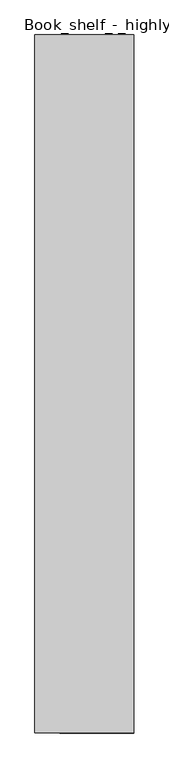
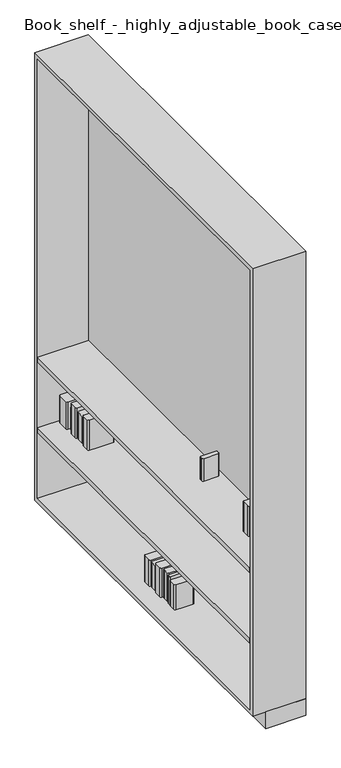
"""IFC4 building model written with IfcOpenShell, lengths in millimetres: furniture geometry."""

from ifc_helpers import new_model, si_unit, point, frame, frame_2d, origin, origin_with_axes, place, context, project, spatial, polyline, circle_curve, trimmed, segment, composite_curve, outline, extrude, source, transform, mapped, element, save


def furniture_61dade96(model_context):
    return source(origin(), model_context, "Body", "SweptSolid", [
        extrude(outline(composite_curve([segment(polyline([(-174.9979766, 273.5343096), (-174.9979766, 313.4842776)]), True, "CONTINUOUS"), segment(trimmed(circle_curve(frame_2d((-168.6479766, 313.4842776)), 6.35), [point((-174.9979766, 313.4842776))], [point((-168.6479766, 319.8342776))], False, "CARTESIAN"), True, "CONTINUOUS"), segment(polyline([(-168.6479766, 319.8342776), (-44.45, 319.8342776)]), True, "CONTINUOUS"), segment(trimmed(circle_curve(frame_2d((-44.45, 313.4842776)), 6.35), [point((-44.45, 319.8342776))], [point((-38.1, 313.4842776))], False, "CARTESIAN"), True, "CONTINUOUS"), segment(polyline([(-38.1, 313.4842776), (-38.1, 273.5343096)]), True, "CONTINUOUS"), segment(trimmed(circle_curve(frame_2d((-44.45, 273.5343096)), 6.35), [point((-38.1, 273.5343096))], [point((-44.45, 267.1843096))], False, "CARTESIAN"), True, "CONTINUOUS"), segment(polyline([(-44.45, 267.1843096), (-168.6479766, 267.1843096)]), True, "CONTINUOUS"), segment(trimmed(circle_curve(frame_2d((-168.6479766, 273.5343096)), 6.35), [point((-168.6479766, 267.1843096))], [point((-174.9979766, 273.5343096))], False, "CARTESIAN"), True, "CONTINUOUS")], self_intersect=False)), frame((0.0, 0.0, 977.8), z_axis=(0.0, 0.0, 1.0), x_axis=(1.0, 0.0, 0.0)), (0.0, 0.0, 1.0), 181.3914823),
        extrude(outline(composite_curve([segment(polyline([(-134.504595, 796.0843096), (-134.504595, 808.7843096)]), True, "CONTINUOUS"), segment(trimmed(circle_curve(frame_2d((-128.154595, 808.7843096)), 6.35), [point((-134.504595, 808.7843096))], [point((-128.154595, 815.1343096))], False, "CARTESIAN"), True, "CONTINUOUS"), segment(polyline([(-128.154595, 815.1343096), (-44.45, 815.1343096)]), True, "CONTINUOUS"), segment(trimmed(circle_curve(frame_2d((-44.45, 808.7843096)), 6.35), [point((-44.45, 815.1343096))], [point((-38.1, 808.7843096))], False, "CARTESIAN"), True, "CONTINUOUS"), segment(polyline([(-38.1, 808.7843096), (-38.1, 796.0843096)]), True, "CONTINUOUS"), segment(trimmed(circle_curve(frame_2d((-44.45, 796.0843096)), 6.35), [point((-38.1, 796.0843096))], [point((-44.45, 789.7343096))], False, "CARTESIAN"), True, "CONTINUOUS"), segment(polyline([(-44.45, 789.7343096), (-128.154595, 789.7343096)]), True, "CONTINUOUS"), segment(trimmed(circle_curve(frame_2d((-128.154595, 796.0843096)), 6.35), [point((-128.154595, 789.7343096))], [point((-134.504595, 796.0843096))], False, "CARTESIAN"), True, "CONTINUOUS")], self_intersect=False)), frame((0.0, 0.0, 977.8), z_axis=(0.0, 0.0, 1.0), x_axis=(1.0, 0.0, 0.0)), (0.0, 0.0, 1.0), 135.8183694),
        extrude(outline(composite_curve([segment(polyline([(-174.9979766, 154.4873472), (-174.9979766, 194.4373151)]), True, "CONTINUOUS"), segment(trimmed(circle_curve(frame_2d((-168.6479766, 194.4373151)), 6.35), [point((-174.9979766, 194.4373151))], [point((-168.6479766, 200.7873151))], False, "CARTESIAN"), True, "CONTINUOUS"), segment(polyline([(-168.6479766, 200.7873151), (-44.45, 200.7873151)]), True, "CONTINUOUS"), segment(trimmed(circle_curve(frame_2d((-44.45, 194.4373151)), 6.35), [point((-44.45, 200.7873151))], [point((-38.1, 194.4373151))], False, "CARTESIAN"), True, "CONTINUOUS"), segment(polyline([(-38.1, 194.4373151), (-38.1, 154.4873472)]), True, "CONTINUOUS"), segment(trimmed(circle_curve(frame_2d((-44.45, 154.4873472)), 6.35), [point((-38.1, 154.4873472))], [point((-44.45, 148.1373472))], False, "CARTESIAN"), True, "CONTINUOUS"), segment(polyline([(-44.45, 148.1373472), (-168.6479766, 148.1373472)]), True, "CONTINUOUS"), segment(trimmed(circle_curve(frame_2d((-168.6479766, 154.4873472)), 6.35), [point((-168.6479766, 148.1373472))], [point((-174.9979766, 154.4873472))], False, "CARTESIAN"), True, "CONTINUOUS")], self_intersect=False)), frame((0.0, 0.0, 977.8), z_axis=(0.0, 0.0, 1.0), x_axis=(1.0, 0.0, 0.0)), (0.0, 0.0, 1.0), 181.3914823),
        extrude(outline(composite_curve([segment(polyline([(-148.9022418, 213.6855624), (-148.9022418, 254.1898725)]), True, "CONTINUOUS"), segment(trimmed(circle_curve(frame_2d((-142.5522418, 254.1898725)), 6.35), [point((-148.9022418, 254.1898725))], [point((-142.5522418, 260.5398725))], False, "CARTESIAN"), True, "CONTINUOUS"), segment(polyline([(-142.5522418, 260.5398725), (-44.45, 260.5398725)]), True, "CONTINUOUS"), segment(trimmed(circle_curve(frame_2d((-44.45, 254.1898725)), 6.35), [point((-44.45, 260.5398725))], [point((-38.1, 254.1898725))], False, "CARTESIAN"), True, "CONTINUOUS"), segment(polyline([(-38.1, 254.1898725), (-38.1, 213.6855624)]), True, "CONTINUOUS"), segment(trimmed(circle_curve(frame_2d((-44.45, 213.6855624)), 6.35), [point((-38.1, 213.6855624))], [point((-44.45, 207.3355624))], False, "CARTESIAN"), True, "CONTINUOUS"), segment(polyline([(-44.45, 207.3355624), (-142.5522418, 207.3355624)]), True, "CONTINUOUS"), segment(trimmed(circle_curve(frame_2d((-142.5522418, 213.6855624)), 6.35), [point((-142.5522418, 207.3355624))], [point((-148.9022418, 213.6855624))], False, "CARTESIAN"), True, "CONTINUOUS")], self_intersect=False)), frame((0.0, 0.0, 977.8), z_axis=(0.0, 0.0, 1.0), x_axis=(1.0, 0.0, 0.0)), (0.0, 0.0, 1.0), 163.8466778),
        extrude(outline(composite_curve([segment(polyline([(-155.6511388, 44.45), (-155.6511388, 48.7119243)]), True, "CONTINUOUS"), segment(trimmed(circle_curve(frame_2d((-149.3011388, 48.7119243)), 6.35), [point((-155.6511388, 48.7119243))], [point((-149.3011388, 55.0619243))], False, "CARTESIAN"), True, "CONTINUOUS"), segment(polyline([(-149.3011388, 55.0619243), (-44.45, 55.0619243)]), True, "CONTINUOUS"), segment(trimmed(circle_curve(frame_2d((-44.45, 48.7119243)), 6.35), [point((-44.45, 55.0619243))], [point((-38.1, 48.7119243))], False, "CARTESIAN"), True, "CONTINUOUS"), segment(polyline([(-38.1, 48.7119243), (-38.1, 44.45)]), True, "CONTINUOUS"), segment(trimmed(circle_curve(frame_2d((-44.45, 44.45)), 6.35), [point((-38.1, 44.45))], [point((-44.45, 38.1))], False, "CARTESIAN"), True, "CONTINUOUS"), segment(polyline([(-44.45, 38.1), (-149.3011388, 38.1)]), True, "CONTINUOUS"), segment(trimmed(circle_curve(frame_2d((-149.3011388, 44.45)), 6.35), [point((-149.3011388, 38.1))], [point((-155.6511388, 44.45))], False, "CARTESIAN"), True, "CONTINUOUS")], self_intersect=False)), frame((0.0, 0.0, 977.8), z_axis=(0.0, 0.0, 1.0), x_axis=(1.0, 0.0, 0.0)), (0.0, 0.0, 1.0), 166.2690481),
        extrude(outline(composite_curve([segment(polyline([(-191.8289872, 93.2744988), (-191.8289872, 133.2244668)]), True, "CONTINUOUS"), segment(trimmed(circle_curve(frame_2d((-185.4789872, 133.2244668)), 6.35), [point((-191.8289872, 133.2244668))], [point((-185.4789872, 139.5744668))], False, "CARTESIAN"), True, "CONTINUOUS"), segment(polyline([(-185.4789872, 139.5744668), (-44.45, 139.5744668)]), True, "CONTINUOUS"), segment(trimmed(circle_curve(frame_2d((-44.45, 133.2244668)), 6.35), [point((-44.45, 139.5744668))], [point((-38.1, 133.2244668))], False, "CARTESIAN"), True, "CONTINUOUS"), segment(polyline([(-38.1, 133.2244668), (-38.1, 93.2744988)]), True, "CONTINUOUS"), segment(trimmed(circle_curve(frame_2d((-44.45, 93.2744988)), 6.35), [point((-38.1, 93.2744988))], [point((-44.45, 86.9244988))], False, "CARTESIAN"), True, "CONTINUOUS"), segment(polyline([(-44.45, 86.9244988), (-185.4789872, 86.9244988)]), True, "CONTINUOUS"), segment(trimmed(circle_curve(frame_2d((-185.4789872, 93.2744988)), 6.35), [point((-185.4789872, 86.9244988))], [point((-191.8289872, 93.2744988))], False, "CARTESIAN"), True, "CONTINUOUS")], self_intersect=False)), frame((0.0, 0.0, 977.8), z_axis=(0.0, 0.0, 1.0), x_axis=(1.0, 0.0, 0.0)), (0.0, 0.0, 1.0), 148.7566688),
        extrude(outline(composite_curve([segment(polyline([(-177.3825869, 67.874514), (-177.3825869, 75.2798723)]), True, "CONTINUOUS"), segment(trimmed(circle_curve(frame_2d((-171.0325869, 75.2798723)), 6.35), [point((-177.3825869, 75.2798723))], [point((-171.0325869, 81.6298723))], False, "CARTESIAN"), True, "CONTINUOUS"), segment(polyline([(-171.0325869, 81.6298723), (-44.45, 81.6298723)]), True, "CONTINUOUS"), segment(trimmed(circle_curve(frame_2d((-44.45, 75.2798723)), 6.35), [point((-44.45, 81.6298723))], [point((-38.1, 75.2798723))], False, "CARTESIAN"), True, "CONTINUOUS"), segment(polyline([(-38.1, 75.2798723), (-38.1, 67.874514)]), True, "CONTINUOUS"), segment(trimmed(circle_curve(frame_2d((-44.45, 67.874514)), 6.35), [point((-38.1, 67.874514))], [point((-44.45, 61.524514))], False, "CARTESIAN"), True, "CONTINUOUS"), segment(polyline([(-44.45, 61.524514), (-171.0325869, 61.524514)]), True, "CONTINUOUS"), segment(trimmed(circle_curve(frame_2d((-171.0325869, 67.874514)), 6.35), [point((-171.0325869, 61.524514))], [point((-177.3825869, 67.874514))], False, "CARTESIAN"), True, "CONTINUOUS")], self_intersect=False)), frame((0.0, 0.0, 977.8), z_axis=(0.0, 0.0, 1.0), x_axis=(1.0, 0.0, 0.0)), (0.0, 0.0, 1.0), 151.8618711),
        extrude(outline(polyline([(0.0, 2124.6), (0.0, 25.4), (-304.8, 25.4), (-304.8, 2124.6), (0.0, 2124.6)])), frame((0.0, 0.0, 952.4), z_axis=(0.0, 0.0, 1.0), x_axis=(1.0, 0.0, 0.0)), (0.0, 0.0, 1.0), 25.4),
        extrude(outline(composite_curve([segment(polyline([(-181.0020996, 119.7389676), (-181.0020996, 160.2432777)]), True, "CONTINUOUS"), segment(trimmed(circle_curve(frame_2d((-174.6520996, 160.2432777)), 6.35), [point((-181.0020996, 160.2432777))], [point((-174.6520996, 166.5932777))], False, "CARTESIAN"), True, "CONTINUOUS"), segment(polyline([(-174.6520996, 166.5932777), (-44.45, 166.5932777)]), True, "CONTINUOUS"), segment(trimmed(circle_curve(frame_2d((-44.45, 160.2432777)), 6.35), [point((-44.45, 166.5932777))], [point((-38.1, 160.2432777))], False, "CARTESIAN"), True, "CONTINUOUS"), segment(polyline([(-38.1, 160.2432777), (-38.1, 119.7389676)]), True, "CONTINUOUS"), segment(trimmed(circle_curve(frame_2d((-44.45, 119.7389676)), 6.35), [point((-38.1, 119.7389676))], [point((-44.45, 113.3889676))], False, "CARTESIAN"), True, "CONTINUOUS"), segment(polyline([(-44.45, 113.3889676), (-174.6520996, 113.3889676)]), True, "CONTINUOUS"), segment(trimmed(circle_curve(frame_2d((-174.6520996, 119.7389676)), 6.35), [point((-174.6520996, 113.3889676))], [point((-181.0020996, 119.7389676))], False, "CARTESIAN"), True, "CONTINUOUS")], self_intersect=False)), frame((0.0, 0.0, 552.4), z_axis=(0.0, 0.0, 1.0), x_axis=(1.0, 0.0, 0.0)), (0.0, 0.0, 1.0), 163.8466778),
        extrude(outline(composite_curve([segment(polyline([(-187.30107, 1955.1650696), (-187.30107, 1995.1150375)]), True, "CONTINUOUS"), segment(trimmed(circle_curve(frame_2d((-180.95107, 1995.1150375)), 6.35), [point((-187.30107, 1995.1150375))], [point((-180.95107, 2001.4650375))], False, "CARTESIAN"), True, "CONTINUOUS"), segment(polyline([(-180.95107, 2001.4650375), (-44.45, 2001.4650375)]), True, "CONTINUOUS"), segment(trimmed(circle_curve(frame_2d((-44.45, 1995.1150375)), 6.35), [point((-44.45, 2001.4650375))], [point((-38.1, 1995.1150375))], False, "CARTESIAN"), True, "CONTINUOUS"), segment(polyline([(-38.1, 1995.1150375), (-38.1, 1955.1650696)]), True, "CONTINUOUS"), segment(trimmed(circle_curve(frame_2d((-44.45, 1955.1650696)), 6.35), [point((-38.1, 1955.1650696))], [point((-44.45, 1948.8150696))], False, "CARTESIAN"), True, "CONTINUOUS"), segment(polyline([(-44.45, 1948.8150696), (-180.95107, 1948.8150696)]), True, "CONTINUOUS"), segment(trimmed(circle_curve(frame_2d((-180.95107, 1955.1650696)), 6.35), [point((-180.95107, 1948.8150696))], [point((-187.30107, 1955.1650696))], False, "CARTESIAN"), True, "CONTINUOUS")], self_intersect=False)), frame((0.0, 0.0, 552.4), z_axis=(0.0, 0.0, 1.0), x_axis=(1.0, 0.0, 0.0)), (0.0, 0.0, 1.0), 181.3914823),
        extrude(outline(composite_curve([segment(polyline([(-186.4012171, 44.45), (-186.4012171, 53.326397)]), True, "CONTINUOUS"), segment(trimmed(circle_curve(frame_2d((-180.0512171, 53.326397)), 6.35), [point((-186.4012171, 53.326397))], [point((-180.0512171, 59.676397))], False, "CARTESIAN"), True, "CONTINUOUS"), segment(polyline([(-180.0512171, 59.676397), (-44.45, 59.676397)]), True, "CONTINUOUS"), segment(trimmed(circle_curve(frame_2d((-44.45, 53.326397)), 6.35), [point((-44.45, 59.676397))], [point((-38.1, 53.326397))], False, "CARTESIAN"), True, "CONTINUOUS"), segment(polyline([(-38.1, 53.326397), (-38.1, 44.45)]), True, "CONTINUOUS"), segment(trimmed(circle_curve(frame_2d((-44.45, 44.45)), 6.35), [point((-38.1, 44.45))], [point((-44.45, 38.1))], False, "CARTESIAN"), True, "CONTINUOUS"), segment(polyline([(-44.45, 38.1), (-180.0512171, 38.1)]), True, "CONTINUOUS"), segment(trimmed(circle_curve(frame_2d((-180.0512171, 44.45)), 6.35), [point((-180.0512171, 38.1))], [point((-186.4012171, 44.45))], False, "CARTESIAN"), True, "CONTINUOUS")], self_intersect=False)), frame((0.0, 0.0, 552.4), z_axis=(0.0, 0.0, 1.0), x_axis=(1.0, 0.0, 0.0)), (0.0, 0.0, 1.0), 209.55),
        extrude(outline(composite_curve([segment(polyline([(-189.1007759, 68.366525), (-189.1007759, 102.4979527)]), True, "CONTINUOUS"), segment(trimmed(circle_curve(frame_2d((-182.7507759, 102.4979527)), 6.35), [point((-189.1007759, 102.4979527))], [point((-182.7507759, 108.8479527))], False, "CARTESIAN"), True, "CONTINUOUS"), segment(polyline([(-182.7507759, 108.8479527), (-44.45, 108.8479527)]), True, "CONTINUOUS"), segment(trimmed(circle_curve(frame_2d((-44.45, 102.4979527)), 6.35), [point((-44.45, 108.8479527))], [point((-38.1, 102.4979527))], False, "CARTESIAN"), True, "CONTINUOUS"), segment(polyline([(-38.1, 102.4979527), (-38.1, 68.366525)]), True, "CONTINUOUS"), segment(trimmed(circle_curve(frame_2d((-44.45, 68.366525)), 6.35), [point((-38.1, 68.366525))], [point((-44.45, 62.016525))], False, "CARTESIAN"), True, "CONTINUOUS"), segment(polyline([(-44.45, 62.016525), (-182.7507759, 62.016525)]), True, "CONTINUOUS"), segment(trimmed(circle_curve(frame_2d((-182.7507759, 68.366525)), 6.35), [point((-182.7507759, 62.016525))], [point((-189.1007759, 68.366525))], False, "CARTESIAN"), True, "CONTINUOUS")], self_intersect=False)), frame((0.0, 0.0, 552.4), z_axis=(0.0, 0.0, 1.0), x_axis=(1.0, 0.0, 0.0)), (0.0, 0.0, 1.0), 193.2682698),
        extrude(outline(composite_curve([segment(polyline([(-172.0035703, 2011.3075348), (-172.0035703, 2024.0075348)]), True, "CONTINUOUS"), segment(trimmed(circle_curve(frame_2d((-165.6535703, 2024.0075348)), 6.35), [point((-172.0035703, 2024.0075348))], [point((-165.6535703, 2030.3575348))], False, "CARTESIAN"), True, "CONTINUOUS"), segment(polyline([(-165.6535703, 2030.3575348), (-44.45, 2030.3575348)]), True, "CONTINUOUS"), segment(trimmed(circle_curve(frame_2d((-44.45, 2024.0075348)), 6.35), [point((-44.45, 2030.3575348))], [point((-38.1, 2024.0075348))], False, "CARTESIAN"), True, "CONTINUOUS"), segment(polyline([(-38.1, 2024.0075348), (-38.1, 2011.3075348)]), True, "CONTINUOUS"), segment(trimmed(circle_curve(frame_2d((-44.45, 2011.3075348)), 6.35), [point((-38.1, 2011.3075348))], [point((-44.45, 2004.9575348))], False, "CARTESIAN"), True, "CONTINUOUS"), segment(polyline([(-44.45, 2004.9575348), (-165.6535703, 2004.9575348)]), True, "CONTINUOUS"), segment(trimmed(circle_curve(frame_2d((-165.6535703, 2011.3075348)), 6.35), [point((-165.6535703, 2004.9575348))], [point((-172.0035703, 2011.3075348))], False, "CARTESIAN"), True, "CONTINUOUS")], self_intersect=False)), frame((0.0, 0.0, 552.4), z_axis=(0.0, 0.0, 1.0), x_axis=(1.0, 0.0, 0.0)), (0.0, 0.0, 1.0), 135.8183694),
        extrude(outline(composite_curve([segment(polyline([(-188.4046355, 2043.8512848), (-188.4046355, 2105.55)]), True, "CONTINUOUS"), segment(trimmed(circle_curve(frame_2d((-182.0546355, 2105.55)), 6.35), [point((-188.4046355, 2105.55))], [point((-182.0546355, 2111.9))], False, "CARTESIAN"), True, "CONTINUOUS"), segment(polyline([(-182.0546355, 2111.9), (-44.45, 2111.9)]), True, "CONTINUOUS"), segment(trimmed(circle_curve(frame_2d((-44.45, 2105.55)), 6.35), [point((-44.45, 2111.9))], [point((-38.1, 2105.55))], False, "CARTESIAN"), True, "CONTINUOUS"), segment(polyline([(-38.1, 2105.55), (-38.1, 2043.8512848)]), True, "CONTINUOUS"), segment(trimmed(circle_curve(frame_2d((-44.45, 2043.8512848)), 6.35), [point((-38.1, 2043.8512848))], [point((-44.45, 2037.5012848))], False, "CARTESIAN"), True, "CONTINUOUS"), segment(polyline([(-44.45, 2037.5012848), (-182.0546355, 2037.5012848)]), True, "CONTINUOUS"), segment(trimmed(circle_curve(frame_2d((-182.0546355, 2043.8512848)), 6.35), [point((-182.0546355, 2037.5012848))], [point((-188.4046355, 2043.8512848))], False, "CARTESIAN"), True, "CONTINUOUS")], self_intersect=False)), frame((0.0, 0.0, 552.4), z_axis=(0.0, 0.0, 1.0), x_axis=(1.0, 0.0, 0.0)), (0.0, 0.0, 1.0), 163.8466778),
        extrude(outline(composite_curve([segment(polyline([(-187.30107, 1834.5150696), (-187.30107, 1874.4650375)]), True, "CONTINUOUS"), segment(trimmed(circle_curve(frame_2d((-180.95107, 1874.4650375)), 6.35), [point((-187.30107, 1874.4650375))], [point((-180.95107, 1880.8150375))], False, "CARTESIAN"), True, "CONTINUOUS"), segment(polyline([(-180.95107, 1880.8150375), (-44.45, 1880.8150375)]), True, "CONTINUOUS"), segment(trimmed(circle_curve(frame_2d((-44.45, 1874.4650375)), 6.35), [point((-44.45, 1880.8150375))], [point((-38.1, 1874.4650375))], False, "CARTESIAN"), True, "CONTINUOUS"), segment(polyline([(-38.1, 1874.4650375), (-38.1, 1834.5150696)]), True, "CONTINUOUS"), segment(trimmed(circle_curve(frame_2d((-44.45, 1834.5150696)), 6.35), [point((-38.1, 1834.5150696))], [point((-44.45, 1828.1650696))], False, "CARTESIAN"), True, "CONTINUOUS"), segment(polyline([(-44.45, 1828.1650696), (-180.95107, 1828.1650696)]), True, "CONTINUOUS"), segment(trimmed(circle_curve(frame_2d((-180.95107, 1834.5150696)), 6.35), [point((-180.95107, 1828.1650696))], [point((-187.30107, 1834.5150696))], False, "CARTESIAN"), True, "CONTINUOUS")], self_intersect=False)), frame((0.0, 0.0, 552.4), z_axis=(0.0, 0.0, 1.0), x_axis=(1.0, 0.0, 0.0)), (0.0, 0.0, 1.0), 181.3914823),
        extrude(outline(composite_curve([segment(polyline([(-181.0020996, 1895.4125122), (-181.0020996, 1935.9168223)]), True, "CONTINUOUS"), segment(trimmed(circle_curve(frame_2d((-174.6520996, 1935.9168223)), 6.35), [point((-181.0020996, 1935.9168223))], [point((-174.6520996, 1942.2668223))], False, "CARTESIAN"), True, "CONTINUOUS"), segment(polyline([(-174.6520996, 1942.2668223), (-44.45, 1942.2668223)]), True, "CONTINUOUS"), segment(trimmed(circle_curve(frame_2d((-44.45, 1935.9168223)), 6.35), [point((-44.45, 1942.2668223))], [point((-38.1, 1935.9168223))], False, "CARTESIAN"), True, "CONTINUOUS"), segment(polyline([(-38.1, 1935.9168223), (-38.1, 1895.4125122)]), True, "CONTINUOUS"), segment(trimmed(circle_curve(frame_2d((-44.45, 1895.4125122)), 6.35), [point((-38.1, 1895.4125122))], [point((-44.45, 1889.0625122))], False, "CARTESIAN"), True, "CONTINUOUS"), segment(polyline([(-44.45, 1889.0625122), (-174.6520996, 1889.0625122)]), True, "CONTINUOUS"), segment(trimmed(circle_curve(frame_2d((-174.6520996, 1895.4125122)), 6.35), [point((-174.6520996, 1889.0625122))], [point((-181.0020996, 1895.4125122))], False, "CARTESIAN"), True, "CONTINUOUS")], self_intersect=False)), frame((0.0, 0.0, 552.4), z_axis=(0.0, 0.0, 1.0), x_axis=(1.0, 0.0, 0.0)), (0.0, 0.0, 1.0), 163.8466778),
        extrude(outline(polyline([(0.0, 2124.6), (0.0, 25.4), (-304.8, 25.4), (-304.8, 2124.6), (0.0, 2124.6)])), frame((0.0, 0.0, 527.0), z_axis=(0.0, 0.0, 1.0), x_axis=(1.0, 0.0, 0.0)), (0.0, 0.0, 1.0), 25.4),
        extrude(outline(polyline([(0.0, 2124.6), (0.0, 25.4000152), (-12.7, 25.4000152), (-12.7, 2124.6), (0.0, 2124.6)])), frame((0.0, 0.0, 127.0), z_axis=(0.0, 0.0, 1.0), x_axis=(1.0, 0.0, 0.0)), (0.0, 0.0, 1.0), 2647.4908752),
        extrude(outline(composite_curve([segment(polyline([(-199.9401921, 957.525), (-199.9401921, 993.1784631)]), True, "CONTINUOUS"), segment(trimmed(circle_curve(frame_2d((-193.5901921, 993.1784631)), 6.35), [point((-199.9401921, 993.1784631))], [point((-193.5901921, 999.5284631))], False, "CARTESIAN"), True, "CONTINUOUS"), segment(polyline([(-193.5901921, 999.5284631), (-94.5880974, 999.5284631)]), True, "CONTINUOUS"), segment(trimmed(circle_curve(frame_2d((-94.5880974, 993.1784631)), 6.35), [point((-94.5880974, 999.5284631))], [point((-88.2380974, 993.1784631))], False, "CARTESIAN"), True, "CONTINUOUS"), segment(polyline([(-88.2380974, 993.1784631), (-88.2380974, 957.525)]), True, "CONTINUOUS"), segment(trimmed(circle_curve(frame_2d((-94.5880974, 957.525)), 6.35), [point((-88.2380974, 957.525))], [point((-94.5880974, 951.175))], False, "CARTESIAN"), True, "CONTINUOUS"), segment(polyline([(-94.5880974, 951.175), (-193.5901921, 951.175)]), True, "CONTINUOUS"), segment(trimmed(circle_curve(frame_2d((-193.5901921, 957.525)), 6.35), [point((-193.5901921, 951.175))], [point((-199.9401921, 957.525))], False, "CARTESIAN"), True, "CONTINUOUS")], self_intersect=False)), frame((0.0, 0.0, 127.0), z_axis=(0.0, 0.0, 1.0), x_axis=(1.0, 0.0, 0.0)), (0.0, 0.0, 1.0), 151.8506516),
        extrude(outline(composite_curve([segment(polyline([(-197.4245661, 1013.9854527), (-197.4245661, 1018.2473771)]), True, "CONTINUOUS"), segment(trimmed(circle_curve(frame_2d((-191.0745661, 1018.2473771)), 6.35), [point((-197.4245661, 1018.2473771))], [point((-191.0745661, 1024.5973771))], False, "CARTESIAN"), True, "CONTINUOUS"), segment(polyline([(-191.0745661, 1024.5973771), (-86.2234274, 1024.5973771)]), True, "CONTINUOUS"), segment(trimmed(circle_curve(frame_2d((-86.2234274, 1018.2473771)), 6.35), [point((-86.2234274, 1024.5973771))], [point((-79.8734274, 1018.2473771))], False, "CARTESIAN"), True, "CONTINUOUS"), segment(polyline([(-79.8734274, 1018.2473771), (-79.8734274, 1013.9854527)]), True, "CONTINUOUS"), segment(trimmed(circle_curve(frame_2d((-86.2234274, 1013.9854527)), 6.35), [point((-79.8734274, 1013.9854527))], [point((-86.2234274, 1007.6354527))], False, "CARTESIAN"), True, "CONTINUOUS"), segment(polyline([(-86.2234274, 1007.6354527), (-191.0745661, 1007.6354527)]), True, "CONTINUOUS"), segment(trimmed(circle_curve(frame_2d((-191.0745661, 1013.9854527)), 6.35), [point((-191.0745661, 1007.6354527))], [point((-197.4245661, 1013.9854527))], False, "CARTESIAN"), True, "CONTINUOUS")], self_intersect=False)), frame((0.0, 0.0, 127.0), z_axis=(0.0, 0.0, 1.0), x_axis=(1.0, 0.0, 0.0)), (0.0, 0.0, 1.0), 166.2690481),
        extrude(outline(composite_curve([segment(polyline([(-205.6861592, 60.325), (-205.6861592, 100.274968)]), True, "CONTINUOUS"), segment(trimmed(circle_curve(frame_2d((-199.3361592, 100.274968)), 6.35), [point((-205.6861592, 100.274968))], [point((-199.3361592, 106.624968))], False, "CARTESIAN"), True, "CONTINUOUS"), segment(polyline([(-199.3361592, 106.624968), (-58.307172, 106.624968)]), True, "CONTINUOUS"), segment(trimmed(circle_curve(frame_2d((-58.307172, 100.274968)), 6.35), [point((-58.307172, 106.624968))], [point((-51.957172, 100.274968))], False, "CARTESIAN"), True, "CONTINUOUS"), segment(polyline([(-51.957172, 100.274968), (-51.957172, 60.325)]), True, "CONTINUOUS"), segment(trimmed(circle_curve(frame_2d((-58.307172, 60.325)), 6.35), [point((-51.957172, 60.325))], [point((-58.307172, 53.975))], False, "CARTESIAN"), True, "CONTINUOUS"), segment(polyline([(-58.307172, 53.975), (-199.3361592, 53.975)]), True, "CONTINUOUS"), segment(trimmed(circle_curve(frame_2d((-199.3361592, 60.325)), 6.35), [point((-199.3361592, 53.975))], [point((-205.6861592, 60.325))], False, "CARTESIAN"), True, "CONTINUOUS")], self_intersect=False)), frame((0.0, 0.0, 127.0), z_axis=(0.0, 0.0, 1.0), x_axis=(1.0, 0.0, 0.0)), (0.0, 0.0, 1.0), 148.7566688),
        extrude(outline(composite_curve([segment(polyline([(-201.5638896, 34.9250152), (-201.5638896, 42.3303734)]), True, "CONTINUOUS"), segment(trimmed(circle_curve(frame_2d((-195.2138896, 42.3303734)), 6.35), [point((-201.5638896, 42.3303734))], [point((-195.2138896, 48.6803734))], False, "CARTESIAN"), True, "CONTINUOUS"), segment(polyline([(-195.2138896, 48.6803734), (-68.6313027, 48.6803734)]), True, "CONTINUOUS"), segment(trimmed(circle_curve(frame_2d((-68.6313027, 42.3303734)), 6.35), [point((-68.6313027, 48.6803734))], [point((-62.2813027, 42.3303734))], False, "CARTESIAN"), True, "CONTINUOUS"), segment(polyline([(-62.2813027, 42.3303734), (-62.2813027, 34.9250152)]), True, "CONTINUOUS"), segment(trimmed(circle_curve(frame_2d((-68.6313027, 34.9250152)), 6.35), [point((-62.2813027, 34.9250152))], [point((-68.6313027, 28.5750152))], False, "CARTESIAN"), True, "CONTINUOUS"), segment(polyline([(-68.6313027, 28.5750152), (-195.2138896, 28.5750152)]), True, "CONTINUOUS"), segment(trimmed(circle_curve(frame_2d((-195.2138896, 34.9250152)), 6.35), [point((-195.2138896, 28.5750152))], [point((-201.5638896, 34.9250152))], False, "CARTESIAN"), True, "CONTINUOUS")], self_intersect=False)), frame((0.0, 0.0, 127.0), z_axis=(0.0, 0.0, 1.0), x_axis=(1.0, 0.0, 0.0)), (0.0, 0.0, 1.0), 151.8618711),
        extrude(outline(polyline([(0.0, 2150.0), (0.0, 0.0), (-228.6, 0.0), (-228.6, 2150.0), (0.0, 2150.0)])), origin_with_axes(), (0.0, 0.0, 1.0), 101.6),
        extrude(outline(composite_curve([segment(polyline([(-192.7413687, 1036.9), (-192.7413687, 1068.65)]), True, "CONTINUOUS"), segment(trimmed(circle_curve(frame_2d((-186.3913687, 1068.65)), 6.35), [point((-192.7413687, 1068.65))], [point((-186.3913687, 1075.0))], False, "CARTESIAN"), True, "CONTINUOUS"), segment(polyline([(-186.3913687, 1075.0), (-53.1948629, 1075.0)]), True, "CONTINUOUS"), segment(trimmed(circle_curve(frame_2d((-53.1948629, 1068.65)), 6.35), [point((-53.1948629, 1075.0))], [point((-46.8448629, 1068.65))], False, "CARTESIAN"), True, "CONTINUOUS"), segment(polyline([(-46.8448629, 1068.65), (-46.8448629, 1036.9)]), True, "CONTINUOUS"), segment(trimmed(circle_curve(frame_2d((-53.1948629, 1036.9)), 6.35), [point((-46.8448629, 1036.9))], [point((-53.1948629, 1030.55))], False, "CARTESIAN"), True, "CONTINUOUS"), segment(polyline([(-53.1948629, 1030.55), (-186.3913687, 1030.55)]), True, "CONTINUOUS"), segment(trimmed(circle_curve(frame_2d((-186.3913687, 1036.9)), 6.35), [point((-186.3913687, 1030.55))], [point((-192.7413687, 1036.9))], False, "CARTESIAN"), True, "CONTINUOUS")], self_intersect=False)), frame((0.0, 0.0, 126.7310239), z_axis=(0.0, 0.0, 1.0), x_axis=(1.0, 0.0, 0.0)), (0.0, 0.0, 1.0), 170.2851068),
        extrude(outline(composite_curve([segment(polyline([(-199.9401921, 1141.675), (-199.9401921, 1177.3284631)]), True, "CONTINUOUS"), segment(trimmed(circle_curve(frame_2d((-193.5901921, 1177.3284631)), 6.35), [point((-199.9401921, 1177.3284631))], [point((-193.5901921, 1183.6784631))], False, "CARTESIAN"), True, "CONTINUOUS"), segment(polyline([(-193.5901921, 1183.6784631), (-94.5880974, 1183.6784631)]), True, "CONTINUOUS"), segment(trimmed(circle_curve(frame_2d((-94.5880974, 1177.3284631)), 6.35), [point((-94.5880974, 1183.6784631))], [point((-88.2380974, 1177.3284631))], False, "CARTESIAN"), True, "CONTINUOUS"), segment(polyline([(-88.2380974, 1177.3284631), (-88.2380974, 1141.675)]), True, "CONTINUOUS"), segment(trimmed(circle_curve(frame_2d((-94.5880974, 1141.675)), 6.35), [point((-88.2380974, 1141.675))], [point((-94.5880974, 1135.325))], False, "CARTESIAN"), True, "CONTINUOUS"), segment(polyline([(-94.5880974, 1135.325), (-193.5901921, 1135.325)]), True, "CONTINUOUS"), segment(trimmed(circle_curve(frame_2d((-193.5901921, 1141.675)), 6.35), [point((-193.5901921, 1135.325))], [point((-199.9401921, 1141.675))], False, "CARTESIAN"), True, "CONTINUOUS")], self_intersect=False)), frame((0.0, 0.0, 126.7310239), z_axis=(0.0, 0.0, 1.0), x_axis=(1.0, 0.0, 0.0)), (0.0, 0.0, 1.0), 151.8506516),
        extrude(outline(composite_curve([segment(polyline([(-205.6861592, 1196.975032), (-205.6861592, 1236.925)]), True, "CONTINUOUS"), segment(trimmed(circle_curve(frame_2d((-199.3361592, 1236.925)), 6.35), [point((-205.6861592, 1236.925))], [point((-199.3361592, 1243.275))], False, "CARTESIAN"), True, "CONTINUOUS"), segment(polyline([(-199.3361592, 1243.275), (-77.4908918, 1243.275)]), True, "CONTINUOUS"), segment(trimmed(circle_curve(frame_2d((-77.4908918, 1236.925)), 6.35), [point((-77.4908918, 1243.275))], [point((-71.1408918, 1236.925))], False, "CARTESIAN"), True, "CONTINUOUS"), segment(polyline([(-71.1408918, 1236.925), (-71.1408918, 1196.975032)]), True, "CONTINUOUS"), segment(trimmed(circle_curve(frame_2d((-77.4908918, 1196.975032)), 6.35), [point((-71.1408918, 1196.975032))], [point((-77.4908918, 1190.625032))], False, "CARTESIAN"), True, "CONTINUOUS"), segment(polyline([(-77.4908918, 1190.625032), (-199.3361592, 1190.625032)]), True, "CONTINUOUS"), segment(trimmed(circle_curve(frame_2d((-199.3361592, 1196.975032)), 6.35), [point((-199.3361592, 1190.625032))], [point((-205.6861592, 1196.975032))], False, "CARTESIAN"), True, "CONTINUOUS")], self_intersect=False)), frame((0.0, 0.0, 126.7310239), z_axis=(0.0, 0.0, 1.0), x_axis=(1.0, 0.0, 0.0)), (0.0, 0.0, 1.0), 157.0434797),
        extrude(outline(composite_curve([segment(polyline([(-205.6861592, 1085.850032), (-205.6861592, 1125.8)]), True, "CONTINUOUS"), segment(trimmed(circle_curve(frame_2d((-199.3361592, 1125.8)), 6.35), [point((-205.6861592, 1125.8))], [point((-199.3361592, 1132.15))], False, "CARTESIAN"), True, "CONTINUOUS"), segment(polyline([(-199.3361592, 1132.15), (-58.307172, 1132.15)]), True, "CONTINUOUS"), segment(trimmed(circle_curve(frame_2d((-58.307172, 1125.8)), 6.35), [point((-58.307172, 1132.15))], [point((-51.957172, 1125.8))], False, "CARTESIAN"), True, "CONTINUOUS"), segment(polyline([(-51.957172, 1125.8), (-51.957172, 1085.850032)]), True, "CONTINUOUS"), segment(trimmed(circle_curve(frame_2d((-58.307172, 1085.850032)), 6.35), [point((-51.957172, 1085.850032))], [point((-58.307172, 1079.500032))], False, "CARTESIAN"), True, "CONTINUOUS"), segment(polyline([(-58.307172, 1079.500032), (-199.3361592, 1079.500032)]), True, "CONTINUOUS"), segment(trimmed(circle_curve(frame_2d((-199.3361592, 1085.850032)), 6.35), [point((-199.3361592, 1079.500032))], [point((-205.6861592, 1085.850032))], False, "CARTESIAN"), True, "CONTINUOUS")], self_intersect=False)), frame((0.0, 0.0, 126.7310239), z_axis=(0.0, 0.0, 1.0), x_axis=(1.0, 0.0, 0.0)), (0.0, 0.0, 1.0), 177.2506516),
        extrude(outline(polyline([(0.0, 2800.0), (2150.0, 2800.0), (2150.0, 101.6), (0.0, 101.6), (0.0, 2800.0)]), holes=[polyline([(25.4000152, 2774.4908752), (25.4000152, 126.7310239), (2124.6, 126.7310239), (2124.6, 2774.4908752), (25.4000152, 2774.4908752)])]), frame((-304.8, 0.0, 0.0), z_axis=(1.0, 0.0, 0.0), x_axis=(0.0, 1.0, 0.0)), (0.0, 0.0, 1.0), 304.8),
    ])


if __name__ == "__main__":
    model = new_model("IFC4")
    model_context = context("Model", 3, world=origin())
    ifc_project = project(units=[si_unit("LENGTHUNIT", "METRE", prefix="MILLI")], contexts=[model_context])
    site = spatial("IfcSite", under=ifc_project)
    building = spatial("IfcBuilding", under=site)
    placement = place(None, origin())
    furniture_shape = furniture_61dade96(model_context)
    element("IfcFurniture", 1, ObjectType="Book_shelf_-_highly_adjustable_book_case_10160 : 3'-0\"w 6'-0\"h", at=placement, inside=building, context=model_context, shape_type="MappedRepresentation", body=[
        mapped(furniture_shape, transform((0.0, 0.0, 0.0), x_axis=(1.0, 0.0, 0.0), y_axis=(0.0, 1.0, 0.0), z_axis=(0.0, 0.0, 1.0))),
    ])
    save(model, "model.ifc")

# Revit data of these elements
# Type "Book_shelf_-_highly_adjustable_book_case_10160 : 3'-0\"w 6'-0\"h"
#   total height = 2.8 m
#   toe kick height = 0.1016 m
#   shelf width = 2.0992 m
#   shelf depth = 0.3048 m
#   shelf 6 bottom = 2.1016 m
#   shelf 5 height = 0.4 m
#   shelf 5 bottom = 1.6762 m
#   shelf 4 height = 0.4 m
#   shelf 4 bottom = 1.2508 m
#   shelf 3 height = 0.4 m
#   shelf 2 height = 0.4 m
#   shelf 1 height = 0.4 m
#   bookcase width = 2.15 m
#   shelf 3 bottom = 0.8254 m
#   shelf 6 = yes
#   shelf 5 = yes
#   shelf 4 = yes
#   shelf 3 = yes
#   shelf 2 books = yes
#   shelf 2 = yes
#   books = yes
#   bookcase back = yes
#   Book5 = book blue
#   Book4 = book red
#   Book3 = book green
#   Book2 = book red
#   Book1 = book light blue
#   Book Shelf = book white
#   Default Elevation = 0
# Element 1 (IfcFurniture, "Book_shelf_-_highly_adjustable_book_case_10160 : 3'-0\"w 6'-0\"h")
#   Materials on its faces: "book red", "book blue", "book green", "book light blue", "book white"
# Materials
#   "book blue": class "Paint", colour RGB 13 13 83, transparency 0
#   "book red": class "Paint", colour RGB 229 30 30, transparency 0
#   "book green": class "Paint", colour RGB 81 104 43, transparency 0
#   "book light blue": class "Paint", colour RGB 81 140 196, transparency 0
#   "book white": class "Paint", colour RGB 211 193 153, transparency 0
